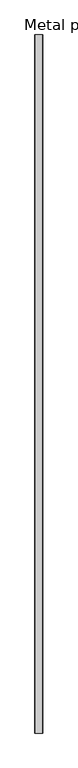
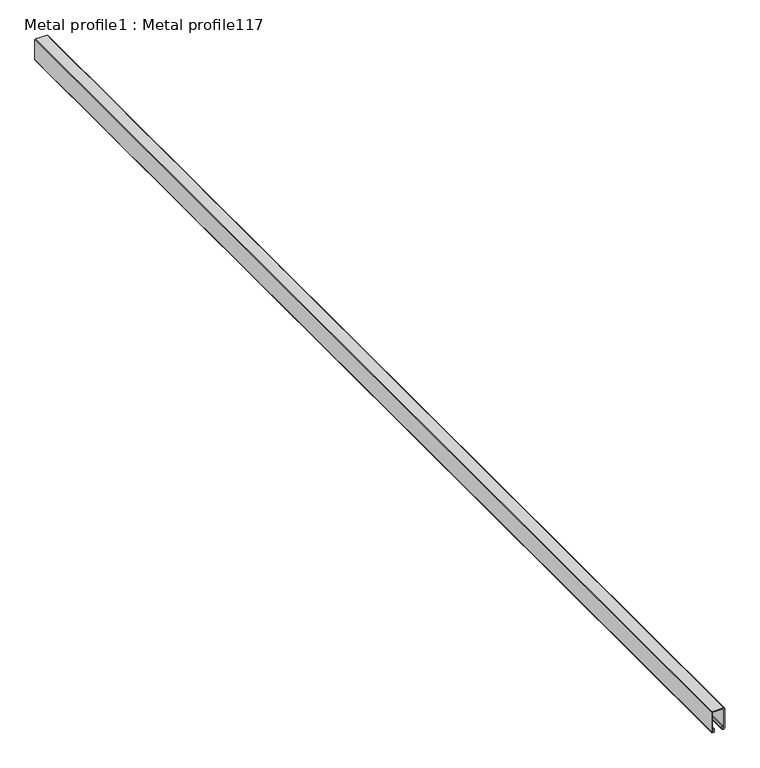
"""IFC4 building model written with IfcOpenShell, lengths in millimetres: proxy geometry, Metal profile1 : Metal profile117."""

from ifc_helpers import new_model, si_unit, point, frame, frame_2d, origin, place, context, project, spatial, polyline, circle_curve, trimmed, segment, composite_curve, outline, extrude, source, transform, mapped, element, save


def metal_profile1_metal_profile117_d3db864a(model_context):
    return source(origin(), model_context, "Body", "SweptSolid", [
        extrude(outline(composite_curve([segment(polyline([(41182.7592895, -7062.8015407), (41182.7592895, -7082.4348882)]), True, "CONTINUOUS"), segment(trimmed(circle_curve(frame_2d((41181.4981858, -7082.4348882)), 1.2611037), [point((41182.7592895, -7082.4348882))], [point((41181.4981858, -7083.6959918))], False, "CARTESIAN"), True, "CONTINUOUS"), segment(polyline([(41181.4981858, -7083.6959918), (41145.9371368, -7083.6959918)]), True, "CONTINUOUS"), segment(trimmed(circle_curve(frame_2d((41145.9371368, -7082.4181446)), 1.2778473), [point((41145.9371368, -7083.6959918))], [point((41144.6592895, -7082.4181446))], False, "CARTESIAN"), True, "CONTINUOUS"), segment(polyline([(41144.6592895, -7082.4181446), (41144.6592895, -7080.2602375)]), True, "CONTINUOUS"), segment(trimmed(circle_curve(frame_2d((41145.9860351, -7080.2602375)), 1.3267456), [point((41144.6592895, -7080.2602375))], [point((41145.9860351, -7078.9334918))], False, "CARTESIAN"), True, "CONTINUOUS"), segment(polyline([(41145.9860351, -7078.9334918), (41151.0592895, -7078.9334918), (41151.0592895, -7080.4334918), (41146.1592895, -7080.4334918), (41146.1592895, -7082.1959918), (41181.2592895, -7082.1959918), (41181.2592895, -7062.9709918), (41146.1592895, -7062.9709918), (41146.1592895, -7064.7334918), (41151.0592895, -7064.7334918), (41151.0592895, -7066.2334918), (41146.0046215, -7066.2334918)]), True, "CONTINUOUS"), segment(trimmed(circle_curve(frame_2d((41146.0046215, -7064.8881599)), 1.345332), [point((41146.0046215, -7066.2334918))], [point((41144.6592895, -7064.8881599))], False, "CARTESIAN"), True, "CONTINUOUS"), segment(polyline([(41144.6592895, -7064.8881599), (41144.6592895, -7062.7274316)]), True, "CONTINUOUS"), segment(trimmed(circle_curve(frame_2d((41145.9157293, -7062.7274316)), 1.2564398), [point((41144.6592895, -7062.7274316))], [point((41145.9157293, -7061.4709918))], False, "CARTESIAN"), True, "CONTINUOUS"), segment(polyline([(41145.9157293, -7061.4709918), (41181.4287407, -7061.4709918)]), True, "CONTINUOUS"), segment(trimmed(circle_curve(frame_2d((41181.4287407, -7062.8015407)), 1.3305488), [point((41181.4287407, -7061.4709918))], [point((41182.7592895, -7062.8015407))], False, "CARTESIAN"), True, "CONTINUOUS")], self_intersect=False)), frame((0.0, 7182.1531721, 0.0), z_axis=(0.0, 1.0, 0.0), x_axis=(0.0, 0.0, 1.0)), (0.0, 0.0, 1.0), 1999.85),
    ])


if __name__ == "__main__":
    model = new_model("IFC4")
    model_context = context("Model", 3, world=origin())
    ifc_project = project(units=[si_unit("LENGTHUNIT", "METRE", prefix="MILLI")], contexts=[model_context])
    site = spatial("IfcSite", under=ifc_project)
    building = spatial("IfcBuilding", under=site)
    placement = place(None, origin())
    metal_profile1_metal_profile117_shape = metal_profile1_metal_profile117_d3db864a(model_context)
    element("IfcBuildingElementProxy", 1, Name="Metal profile1 : Metal profile117", ObjectType="Metal profile1 : Metal profile117", at=placement, inside=building, context=model_context, shape_type="MappedRepresentation", body=[
        mapped(metal_profile1_metal_profile117_shape, transform((0.0, 0.0, 0.0), x_axis=(1.0, 0.0, 0.0), y_axis=(0.0, 1.0, 0.0), z_axis=(0.0, 0.0, 1.0))),
    ])
    save(model, "model.ifc")

# Revit data of these elements
# Type "Metal profile1 : Metal profile117"
#   NameOverride = "Metal profile117"
# Element 1 (IfcBuildingElementProxy, "Metal profile1 : Metal profile117")
#   Materials on its faces: "CRL U-CHANNEL GRUC5 SERIES FOR 1/2\" GLASS TO SPAN CONTINUOUSLY ACROSS AT LEAST 3 PANELS"
# Materials
#   "CRL U-CHANNEL GRUC5 SERIES FOR 1/2\" GLASS TO SPAN CONTINUOUSLY ACROSS AT LEAST 3 PANELS": class "Unassigned", colour RGB 128 128 128, transparency 0, Cost = 0
